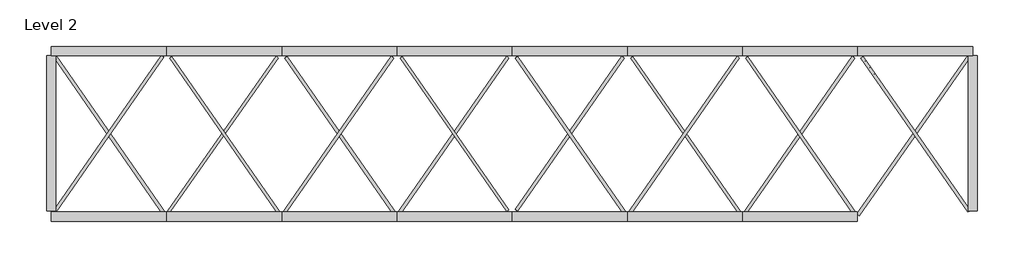
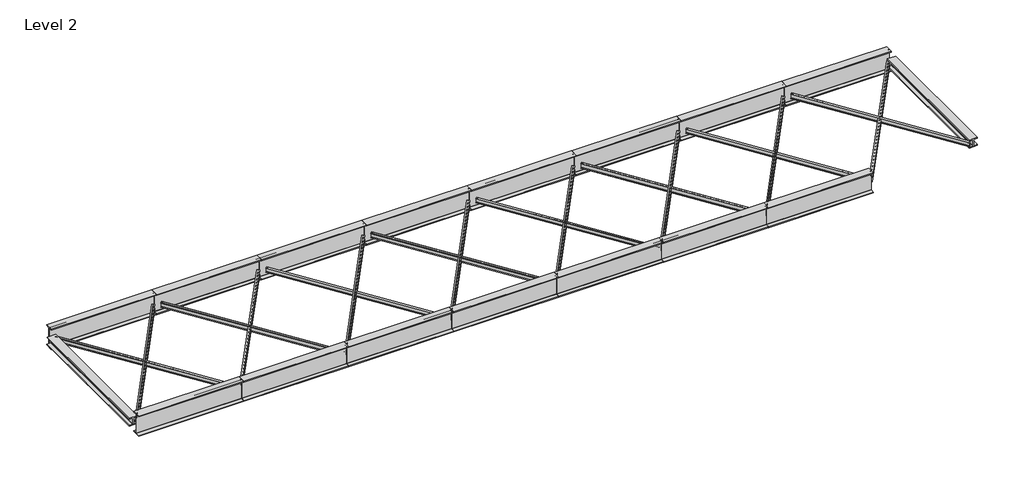
# One storey: 18 members, 15 beams.
"""IFC4 building model written with IfcOpenShell, lengths in millimetres."""

import ifcopenshell
import ifcopenshell.guid

model = None  # the IFC model being written
_history = None  # IfcOwnerHistory: only IFC2X3 demands one
_inside = {}  # id of a spatial element -> (the spatial element, [elements in it])
_under = {}  # id of a project, library or spatial element -> (it, [spatial elements below it])
_declared = {}  # id of a project -> (the project, [libraries it declares])
_typed = {}  # id of a type object -> (the type object, [elements of that type])
_made_of = {}  # id of a material, layer set ... -> (it, [elements and type objects made of it])


def new_model(schema):
    """Start an empty IFC model of exactly this schema.

    Asked for "IFC4X3", IfcOpenShell would pick the latest addendum, in which some entities
    have other attributes; the version numbers below select the first issue.
    IFC2X3 requires an IfcOwnerHistory on every rooted entity: one is made here for all.
    """
    global model, _history
    if schema == "IFC4X3":
        model = ifcopenshell.file(schema_version=(4, 3, 0, 0))
    else:
        model = ifcopenshell.file(schema=schema)
    _inside.clear()
    _under.clear()
    _declared.clear()
    _typed.clear()
    _made_of.clear()
    _history = None
    if model.schema == "IFC2X3":
        org = make("IfcOrganization", Name="unknown")
        user = make(
            "IfcPersonAndOrganization",
            ThePerson=make("IfcPerson", FamilyName="unknown"),
            TheOrganization=org,
        )
        app = make(
            "IfcApplication",
            ApplicationDeveloper=org,
            Version="unknown",
            ApplicationFullName="unknown",
            ApplicationIdentifier="unknown",
        )
        _history = make(
            "IfcOwnerHistory",
            OwningUser=user,
            OwningApplication=app,
            ChangeAction="ADDED",
            CreationDate=0,
        )
    return model


def make(cls, **values):
    """One entity of the class cls with the attributes given. An attribute that is None is left unset."""
    return model.create_entity(
        cls, **{name: value for name, value in values.items() if value is not None}
    )


def rooted(cls, **values):
    """An entity with a GlobalId (a new one), such as an element, a storey or a relation."""
    return make(cls, GlobalId=ifcopenshell.guid.new(), OwnerHistory=_history, **values)


def si_unit(unit_type, name, prefix=None):
    """IfcSIUnit, for example si_unit("LENGTHUNIT", "METRE", prefix="MILLI")."""
    return make("IfcSIUnit", UnitType=unit_type, Prefix=prefix, Name=name)


def assignment(units):
    """IfcUnitAssignment: the units of a project."""
    return None if units is None else make("IfcUnitAssignment", Units=units)


def point(xyz):
    """IfcCartesianPoint."""
    return None if xyz is None else make("IfcCartesianPoint", Coordinates=xyz)


def direction(xyz):
    """IfcDirection."""
    return None if xyz is None else make("IfcDirection", DirectionRatios=xyz)


def frame(location, z_axis=None, x_axis=None):
    """IfcAxis2Placement3D, a coordinate frame: its origin and axes. An axis left out is left unset."""
    return make(
        "IfcAxis2Placement3D",
        Location=point(location),
        Axis=direction(z_axis),
        RefDirection=direction(x_axis),
    )


def frame_2d(location, x_axis=None):
    """IfcAxis2Placement2D, a coordinate frame in the plane: its origin and x axis."""
    return make(
        "IfcAxis2Placement2D", Location=point(location), RefDirection=direction(x_axis)
    )


def origin():
    """The frame at (0, 0, 0) with its axes left unset."""
    return frame((0.0, 0.0, 0.0))


def place(relative_to, where):
    """IfcLocalPlacement: puts the frame where relative to a parent placement (None: the world)."""
    return make(
        "IfcLocalPlacement", PlacementRelTo=relative_to, RelativePlacement=where
    )


def context(
    kind, dimensions, precision=None, world=None, true_north=None, identifier=None
):
    """IfcGeometricRepresentationContext, for example the 3D "Model" context."""
    return make(
        "IfcGeometricRepresentationContext",
        ContextIdentifier=identifier,
        ContextType=kind,
        CoordinateSpaceDimension=dimensions,
        Precision=precision,
        WorldCoordinateSystem=world,
        TrueNorth=true_north,
    )


def project(units=None, contexts=None):
    """IfcProject with its units and contexts."""
    return rooted(
        "IfcProject",
        Name="project",
        RepresentationContexts=contexts,
        UnitsInContext=assignment(units),
    )


def spatial(cls, under=None, at=None, **own):
    """A site, building, storey or space (cls), placed at a placement, below another one or the project."""
    s = rooted(cls, ObjectPlacement=at, **own)
    if under is not None:
        _under.setdefault(under.id(), (under, []))[1].append(s)
    return s


def polyline(points):
    """IfcPolyline through the points."""
    return make("IfcPolyline", Points=[point(p) for p in points])


def circle_curve(where, radius):
    """IfcCircle in the frame where."""
    return make("IfcCircle", Position=where, Radius=radius)


def trimmed(basis, trim1, trim2, sense, master):
    """IfcTrimmedCurve: the piece of a basis curve between two trims."""
    return make(
        "IfcTrimmedCurve",
        BasisCurve=basis,
        Trim1=trim1,
        Trim2=trim2,
        SenseAgreement=sense,
        MasterRepresentation=master,
    )


def segment(curve, same_sense, transition):
    """IfcCompositeCurveSegment."""
    return make(
        "IfcCompositeCurveSegment",
        Transition=transition,
        SameSense=same_sense,
        ParentCurve=curve,
    )


def composite_curve(segments, self_intersect=None):
    """IfcCompositeCurve: segments joined end to end."""
    return make("IfcCompositeCurve", Segments=segments, SelfIntersect=self_intersect)


def outline(outer, holes=None, kind="AREA"):
    """IfcArbitraryClosedProfileDef: a profile drawn as a closed curve; with holes, ...WithVoids."""
    if holes is None:
        return make("IfcArbitraryClosedProfileDef", ProfileType=kind, OuterCurve=outer)
    return make(
        "IfcArbitraryProfileDefWithVoids",
        ProfileType=kind,
        OuterCurve=outer,
        InnerCurves=holes,
    )


def extrude(swept, where, along, depth):
    """IfcExtrudedAreaSolid: the profile swept, set in the frame where, extruded along a direction by depth."""
    return make(
        "IfcExtrudedAreaSolid",
        SweptArea=swept,
        Position=where,
        ExtrudedDirection=direction(along),
        Depth=depth,
    )


def shape(context_of_items, identifier, shape_type, items):
    """IfcShapeRepresentation: the items that make up one representation, for example the "Body"."""
    return make(
        "IfcShapeRepresentation",
        ContextOfItems=context_of_items,
        RepresentationIdentifier=identifier,
        RepresentationType=shape_type,
        Items=items,
    )


def source(mapping_origin, context_of_items, identifier, shape_type, items):
    """IfcRepresentationMap: a shape defined once, which mapped items show again and again."""
    return make(
        "IfcRepresentationMap",
        MappingOrigin=mapping_origin,
        MappedRepresentation=shape(context_of_items, identifier, shape_type, items),
    )


def transform(
    local_origin,
    x_axis=None,
    y_axis=None,
    z_axis=None,
    scale=None,
    scale2=None,
    scale3=None,
    uniform=True,
):
    """IfcCartesianTransformationOperator3D, or its non-uniform kind. x_axis, y_axis, z_axis: its Axis1, 2, 3."""
    if uniform:
        return make(
            "IfcCartesianTransformationOperator3D",
            Axis1=direction(x_axis),
            Axis2=direction(y_axis),
            LocalOrigin=point(local_origin),
            Scale=scale,
            Axis3=direction(z_axis),
        )
    return make(
        "IfcCartesianTransformationOperator3DnonUniform",
        Axis1=direction(x_axis),
        Axis2=direction(y_axis),
        LocalOrigin=point(local_origin),
        Scale=scale,
        Axis3=direction(z_axis),
        Scale2=scale2,
        Scale3=scale3,
    )


def mapped(mapping_source, mapping_target):
    """IfcMappedItem: shows the shape of a source again, moved by a transform."""
    return make(
        "IfcMappedItem", MappingSource=mapping_source, MappingTarget=mapping_target
    )


def made_of(thing, what):
    """Note that an element or type object is made of a material, layer set ...; save() writes the relation."""
    if what is not None:
        _made_of.setdefault(what.id(), (what, []))[1].append(thing)
    return thing


def element(
    cls,
    number,
    at=None,
    inside=None,
    cuts=None,
    type_object=None,
    material=None,
    context=None,
    identifier="Body",
    shape_type=None,
    held_by="IfcProductDefinitionShape",
    body=None,
    shapes=None,
    **own,
):
    """One element of the class cls, such as IfcWall. Its Tag is "e" and its number.

    at: its placement. inside: the storey or other place that contains it. cuts: it is an
    opening in that element (IfcRelVoidsElement). A single representation is given by context,
    identifier, shape_type and body (its items); several are given by shapes. held_by: the class
    of the entity that holds the representations. save() writes the other relations.
    """
    e = rooted(cls, Tag="e%d" % number, ObjectPlacement=at, **own)
    if body is not None:
        shapes = [shape(context, identifier, shape_type, body)]
    if shapes is not None:
        e.Representation = make(held_by, Representations=shapes)
    if inside is not None:
        _inside.setdefault(inside.id(), (inside, []))[1].append(e)
    if cuts is not None:
        rooted(
            "IfcRelVoidsElement", RelatingBuildingElement=cuts, RelatedOpeningElement=e
        )
    if type_object is not None:
        _typed.setdefault(type_object.id(), (type_object, []))[1].append(e)
    return made_of(e, material)


def aggregate(whole, parts):
    """IfcRelAggregates: a whole, such as a stair, and the parts it consists of."""
    return rooted("IfcRelAggregates", RelatingObject=whole, RelatedObjects=parts)


def save(model, path):
    """Write the relations noted so far, then the file.

    IfcRelAggregates (storeys below a building ...), IfcRelContainedInSpatialStructure (elements
    in a storey), IfcRelDefinesByType, IfcRelAssociatesMaterial and IfcRelDeclares: one each for
    every whole, place, type object, material and project.
    """
    for whole, parts in _under.values():
        aggregate(whole, parts)
    for where, things in _inside.values():
        rooted(
            "IfcRelContainedInSpatialStructure",
            RelatedElements=things,
            RelatingStructure=where,
        )
    for kind, things in _typed.values():
        rooted("IfcRelDefinesByType", RelatedObjects=things, RelatingType=kind)
    for what, things in _made_of.values():
        rooted("IfcRelAssociatesMaterial", RelatedObjects=things, RelatingMaterial=what)
    for by, libraries in _declared.values():
        rooted("IfcRelDeclares", RelatingContext=by, RelatedDefinitions=libraries)
    model.write(path)


def wwf_welded_wide_flange_wwf55x402_e03ff242(model_context):
    return source(origin(), model_context, "Body", "SweptSolid", [
        extrude(outline(polyline([(274.955, -649.986), (274.955, -700.024), (-274.955, -700.024), (-274.955, -649.986), (-19.05, -649.986), (-8.001, -638.937), (-8.001, 638.937), (-19.05, 649.986), (-274.955, 649.986), (-274.955, 700.024), (274.955, 700.024), (274.955, 649.986), (19.05, 649.986), (8.001, 638.937), (8.001, -638.937), (19.05, -649.986), (274.955, -649.986)])), frame((-3472.2183929, 0.0, 0.0), z_axis=(1.0, 0.0, 0.0), x_axis=(0.0, 1.0, 0.0)), (0.0, 0.0, 1.0), 6944.4367858),
    ])


def wwf_welded_wide_flange_wwf55x402_453157a7(model_context):
    return source(origin(), model_context, "Body", "SweptSolid", [
        extrude(outline(polyline([(274.955, -649.986), (274.955, -700.024), (-274.955, -700.024), (-274.955, -649.986), (-19.05, -649.986), (-8.001, -638.937), (-8.001, 638.937), (-19.05, 649.986), (-274.955, 649.986), (-274.955, 700.024), (274.955, 700.024), (274.955, 649.986), (19.05, 649.986), (8.001, 638.937), (8.001, -638.937), (19.05, -649.986), (274.955, -649.986)])), frame((-3472.218169, 0.0, 0.0), z_axis=(1.0, 0.0, 0.0), x_axis=(0.0, 1.0, 0.0)), (0.0, 0.0, 1.0), 6944.436338),
    ])


def wwf_welded_wide_flange_wwf55x402_a9ee8206(model_context):
    return source(origin(), model_context, "Body", "SweptSolid", [
        extrude(outline(polyline([(274.955, -649.986), (274.955, -700.024), (-274.955, -700.024), (-274.955, -649.986), (-19.05, -649.986), (-8.001, -638.937), (-8.001, 638.937), (-19.05, 649.986), (-274.955, 649.986), (-274.955, 700.024), (274.955, 700.024), (274.955, 649.986), (19.05, 649.986), (8.001, 638.937), (8.001, -638.937), (19.05, -649.986), (274.955, -649.986)])), frame((-3459.5263379, 0.0, 0.0), z_axis=(1.0, 0.0, 0.0), x_axis=(0.0, 1.0, 0.0)), (0.0, 0.0, 1.0), 6931.7526763),
    ])


def wwf_welded_wide_flange_wwf55x402_d8a73b6f(model_context):
    return source(origin(), model_context, "Body", "SweptSolid", [
        extrude(outline(polyline([(274.955, -649.986), (274.955, -700.024), (-274.955, -700.024), (-274.955, -649.986), (-19.05, -649.986), (-8.001, -638.937), (-8.001, 638.937), (-19.05, 649.986), (-274.955, 649.986), (-274.955, 700.024), (274.955, 700.024), (274.955, 649.986), (19.05, 649.986), (8.001, 638.937), (8.001, -638.937), (19.05, -649.986), (274.955, -649.986)])), frame((-3472.2200653, 0.0, 0.0), z_axis=(1.0, 0.0, 0.0), x_axis=(0.0, 1.0, 0.0)), (0.0, 0.0, 1.0), 6931.74013),
    ])


def wwf_welded_wide_flange_wwf55x402_ad15bced(model_context):
    return source(origin(), model_context, "Body", "SweptSolid", [
        extrude(outline(polyline([(274.955, -649.986), (274.955, -700.024), (-274.955, -700.024), (-274.955, -649.986), (-19.05, -649.986), (-8.001, -638.937), (-8.001, 638.937), (-19.05, 649.986), (-274.955, 649.986), (-274.955, 700.024), (274.955, 700.024), (274.955, 649.986), (19.05, 649.986), (8.001, 638.937), (8.001, -638.937), (19.05, -649.986), (274.955, -649.986)])), frame((-3459.52714, 0.0, 0.0), z_axis=(1.0, 0.0, 0.0), x_axis=(0.0, 1.0, 0.0)), (0.0, 0.0, 1.0), 6919.0542799),
    ])


def wwf_welded_wide_flange_wwf55x402_d46538ab(model_context):
    return source(origin(), model_context, "Body", "SweptSolid", [
        extrude(outline(polyline([(274.955, -649.986), (274.955, -700.024), (-274.955, -700.024), (-274.955, -649.986), (-19.05, -649.986), (-8.001, -638.937), (-8.001, 638.937), (-19.05, 649.986), (-274.955, 649.986), (-274.955, 700.024), (274.955, 700.024), (274.955, 649.986), (19.05, 649.986), (8.001, 638.937), (8.001, -638.937), (19.05, -649.986), (274.955, -649.986)])), frame((-3472.22503, 0.0, 0.0), z_axis=(1.0, 0.0, 0.0), x_axis=(0.0, 1.0, 0.0)), (0.0, 0.0, 1.0), 6931.7500593),
    ])


def wwf_welded_wide_flange_wwf55x402_6292d54f(model_context):
    return source(origin(), model_context, "Body", "SweptSolid", [
        extrude(outline(polyline([(274.955, -649.986), (274.955, -700.024), (-274.955, -700.024), (-274.955, -649.986), (-19.05, -649.986), (-8.001, -638.937), (-8.001, 638.937), (-19.05, 649.986), (-274.955, 649.986), (-274.955, 700.024), (274.955, 700.024), (274.955, 649.986), (19.05, 649.986), (8.001, 638.937), (8.001, -638.937), (19.05, -649.986), (274.955, -649.986)])), frame((-3472.2230903, 0.0, 0.0), z_axis=(1.0, 0.0, 0.0), x_axis=(0.0, 1.0, 0.0)), (0.0, 0.0, 1.0), 6931.7461799),
    ])


def wwf_welded_wide_flange_wwf55x402_e70519e9(model_context):
    return source(origin(), model_context, "Body", "SweptSolid", [
        extrude(outline(polyline([(274.955, -649.986), (274.955, -700.024), (-274.955, -700.024), (-274.955, -649.986), (-19.05, -649.986), (-8.001, -638.937), (-8.001, 638.937), (-19.05, 649.986), (-274.955, 649.986), (-274.955, 700.024), (274.955, 700.024), (274.955, 649.986), (19.05, 649.986), (8.001, 638.937), (8.001, -638.937), (19.05, -649.986), (274.955, -649.986)])), frame((-3459.5195507, 0.0, 0.0), z_axis=(1.0, 0.0, 0.0), x_axis=(0.0, 1.0, 0.0)), (0.0, 0.0, 1.0), 6931.739102),
    ])


def ub_universal_beams_ub305x165x40_783ac592(model_context):
    return source(origin(), model_context, "Body", "SweptSolid", [
        extrude(outline(composite_curve([segment(polyline([(82.5, -141.5), (82.5, -151.7), (-82.5, -151.7), (-82.5, -141.5), (-11.9, -141.5)]), True, "CONTINUOUS"), segment(trimmed(circle_curve(frame_2d((-11.9, -132.6)), 8.9), [point((-11.9, -141.5))], [point((-3.0, -132.6))], True, "CARTESIAN"), True, "CONTINUOUS"), segment(polyline([(-3.0, -132.6), (-3.0, 132.6)]), True, "CONTINUOUS"), segment(trimmed(circle_curve(frame_2d((-11.9, 132.6)), 8.9), [point((-3.0, 132.6))], [point((-11.9, 141.5))], True, "CARTESIAN"), True, "CONTINUOUS"), segment(polyline([(-11.9, 141.5), (-82.5, 141.5), (-82.5, 151.7), (82.5, 151.7), (82.5, 141.5), (11.9, 141.5)]), True, "CONTINUOUS"), segment(trimmed(circle_curve(frame_2d((11.9, 132.6)), 8.9), [point((11.9, 141.5))], [point((3.0, 132.6))], True, "CARTESIAN"), True, "CONTINUOUS"), segment(polyline([(3.0, 132.6), (3.0, -132.6)]), True, "CONTINUOUS"), segment(trimmed(circle_curve(frame_2d((11.9, -132.6)), 8.9), [point((3.0, -132.6))], [point((11.9, -141.5))], True, "CARTESIAN"), True, "CONTINUOUS"), segment(polyline([(11.9, -141.5), (82.5, -141.5)]), True, "CONTINUOUS")], self_intersect=False)), frame((-5697.7, 0.0, 0.0), z_axis=(1.0, 0.0, 0.0), x_axis=(0.0, 1.0, 0.0)), (0.0, 0.0, 1.0), 11670.0),
    ])


def ub_universal_beams_ub305x165x40_9e40c5b6(model_context):
    return source(origin(), model_context, "Body", "SweptSolid", [
        extrude(outline(composite_curve([segment(polyline([(82.5, -141.5), (82.5, -151.7), (-82.5, -151.7), (-82.5, -141.5), (-11.9, -141.5)]), True, "CONTINUOUS"), segment(trimmed(circle_curve(frame_2d((-11.9, -132.6)), 8.9), [point((-11.9, -141.5))], [point((-3.0, -132.6))], True, "CARTESIAN"), True, "CONTINUOUS"), segment(polyline([(-3.0, -132.6), (-3.0, 132.6)]), True, "CONTINUOUS"), segment(trimmed(circle_curve(frame_2d((-11.9, 132.6)), 8.9), [point((-3.0, 132.6))], [point((-11.9, 141.5))], True, "CARTESIAN"), True, "CONTINUOUS"), segment(polyline([(-11.9, 141.5), (-82.5, 141.5), (-82.5, 151.7), (82.5, 151.7), (82.5, 141.5), (11.9, 141.5)]), True, "CONTINUOUS"), segment(trimmed(circle_curve(frame_2d((11.9, 132.6)), 8.9), [point((11.9, 141.5))], [point((3.0, 132.6))], True, "CARTESIAN"), True, "CONTINUOUS"), segment(polyline([(3.0, 132.6), (3.0, -132.6)]), True, "CONTINUOUS"), segment(trimmed(circle_curve(frame_2d((11.9, -132.6)), 8.9), [point((3.0, -132.6))], [point((11.9, -141.5))], True, "CARTESIAN"), True, "CONTINUOUS"), segment(polyline([(11.9, -141.5), (82.5, -141.5)]), True, "CONTINUOUS")], self_intersect=False)), frame((-5682.6, 0.0, 0.0), z_axis=(1.0, 0.0, 0.0), x_axis=(0.0, 1.0, 0.0)), (0.0, 0.0, 1.0), 11365.2),
    ])


def ub_universal_beams_ub305x165x40_3335d084(model_context):
    return source(origin(), model_context, "Body", "SweptSolid", [
        extrude(outline(composite_curve([segment(polyline([(82.5, -141.5), (82.5, -151.7), (-82.5, -151.7), (-82.5, -141.5), (-11.9, -141.5)]), True, "CONTINUOUS"), segment(trimmed(circle_curve(frame_2d((-11.9, -132.6)), 8.9), [point((-11.9, -141.5))], [point((-3.0, -132.6))], True, "CARTESIAN"), True, "CONTINUOUS"), segment(polyline([(-3.0, -132.6), (-3.0, 132.6)]), True, "CONTINUOUS"), segment(trimmed(circle_curve(frame_2d((-11.9, 132.6)), 8.9), [point((-3.0, 132.6))], [point((-11.9, 141.5))], True, "CARTESIAN"), True, "CONTINUOUS"), segment(polyline([(-11.9, 141.5), (-82.5, 141.5), (-82.5, 151.7), (82.5, 151.7), (82.5, 141.5), (11.9, 141.5)]), True, "CONTINUOUS"), segment(trimmed(circle_curve(frame_2d((11.9, 132.6)), 8.9), [point((11.9, 141.5))], [point((3.0, 132.6))], True, "CARTESIAN"), True, "CONTINUOUS"), segment(polyline([(3.0, 132.6), (3.0, -132.6)]), True, "CONTINUOUS"), segment(trimmed(circle_curve(frame_2d((11.9, -132.6)), 8.9), [point((3.0, -132.6))], [point((11.9, -141.5))], True, "CARTESIAN"), True, "CONTINUOUS"), segment(polyline([(11.9, -141.5), (82.5, -141.5)]), True, "CONTINUOUS")], self_intersect=False)), frame((-5955.8, 0.0, 0.0), z_axis=(1.0, 0.0, 0.0), x_axis=(0.0, 1.0, 0.0)), (0.0, 0.0, 1.0), 11638.4),
    ])


def ub_universal_beams_ub305x165x40_035d116d(model_context):
    return source(origin(), model_context, "Body", "SweptSolid", [
        extrude(outline(composite_curve([segment(polyline([(82.5, -141.5), (82.5, -151.7), (-82.5, -151.7), (-82.5, -141.5), (-11.9, -141.5)]), True, "CONTINUOUS"), segment(trimmed(circle_curve(frame_2d((-11.9, -132.6)), 8.9), [point((-11.9, -141.5))], [point((-3.0, -132.6))], True, "CARTESIAN"), True, "CONTINUOUS"), segment(polyline([(-3.0, -132.6), (-3.0, 132.6)]), True, "CONTINUOUS"), segment(trimmed(circle_curve(frame_2d((-11.9, 132.6)), 8.9), [point((-3.0, 132.6))], [point((-11.9, 141.5))], True, "CARTESIAN"), True, "CONTINUOUS"), segment(polyline([(-11.9, 141.5), (-82.5, 141.5), (-82.5, 151.7), (82.5, 151.7), (82.5, 141.5), (11.9, 141.5)]), True, "CONTINUOUS"), segment(trimmed(circle_curve(frame_2d((11.9, 132.6)), 8.9), [point((11.9, 141.5))], [point((3.0, 132.6))], True, "CARTESIAN"), True, "CONTINUOUS"), segment(polyline([(3.0, 132.6), (3.0, -132.6)]), True, "CONTINUOUS"), segment(trimmed(circle_curve(frame_2d((11.9, -132.6)), 8.9), [point((3.0, -132.6))], [point((11.9, -141.5))], True, "CARTESIAN"), True, "CONTINUOUS"), segment(polyline([(11.9, -141.5), (82.5, -141.5)]), True, "CONTINUOUS")], self_intersect=False)), frame((-5621.65, 0.0, 0.0), z_axis=(1.0, 0.0, 0.0), x_axis=(0.0, 1.0, 0.0)), (0.0, 0.0, 1.0), 11577.5),
    ])


def ub_universal_beams_ub305x165x40_793367f0(model_context):
    return source(origin(), model_context, "Body", "SweptSolid", [
        extrude(outline(composite_curve([segment(polyline([(82.5, -141.5), (82.5, -151.7), (-82.5, -151.7), (-82.5, -141.5), (-11.9, -141.5)]), True, "CONTINUOUS"), segment(trimmed(circle_curve(frame_2d((-11.9, -132.6)), 8.9), [point((-11.9, -141.5))], [point((-3.0, -132.6))], True, "CARTESIAN"), True, "CONTINUOUS"), segment(polyline([(-3.0, -132.6), (-3.0, 132.6)]), True, "CONTINUOUS"), segment(trimmed(circle_curve(frame_2d((-11.9, 132.6)), 8.9), [point((-3.0, 132.6))], [point((-11.9, 141.5))], True, "CARTESIAN"), True, "CONTINUOUS"), segment(polyline([(-11.9, 141.5), (-82.5, 141.5), (-82.5, 151.7), (82.5, 151.7), (82.5, 141.5), (11.9, 141.5)]), True, "CONTINUOUS"), segment(trimmed(circle_curve(frame_2d((11.9, 132.6)), 8.9), [point((11.9, 141.5))], [point((3.0, 132.6))], True, "CARTESIAN"), True, "CONTINUOUS"), segment(polyline([(3.0, 132.6), (3.0, -132.6)]), True, "CONTINUOUS"), segment(trimmed(circle_curve(frame_2d((11.9, -132.6)), 8.9), [point((3.0, -132.6))], [point((11.9, -141.5))], True, "CARTESIAN"), True, "CONTINUOUS"), segment(polyline([(11.9, -141.5), (82.5, -141.5)]), True, "CONTINUOUS")], self_intersect=False)), frame((-5600.7, 0.0, 0.0), z_axis=(1.0, 0.0, 0.0), x_axis=(0.0, 1.0, 0.0)), (0.0, 0.0, 1.0), 11654.3),
    ])


def ub_universal_beams_ub305x165x40_c2663d37(model_context):
    return source(origin(), model_context, "Body", "SweptSolid", [
        extrude(outline(composite_curve([segment(polyline([(82.5, -141.5), (82.5, -151.7), (-82.5, -151.7), (-82.5, -141.5), (-11.9, -141.5)]), True, "CONTINUOUS"), segment(trimmed(circle_curve(frame_2d((-11.9, -132.6)), 8.9), [point((-11.9, -141.5))], [point((-3.0, -132.6))], True, "CARTESIAN"), True, "CONTINUOUS"), segment(polyline([(-3.0, -132.6), (-3.0, 132.6)]), True, "CONTINUOUS"), segment(trimmed(circle_curve(frame_2d((-11.9, 132.6)), 8.9), [point((-3.0, 132.6))], [point((-11.9, 141.5))], True, "CARTESIAN"), True, "CONTINUOUS"), segment(polyline([(-11.9, 141.5), (-82.5, 141.5), (-82.5, 151.7), (82.5, 151.7), (82.5, 141.5), (11.9, 141.5)]), True, "CONTINUOUS"), segment(trimmed(circle_curve(frame_2d((11.9, 132.6)), 8.9), [point((11.9, 141.5))], [point((3.0, 132.6))], True, "CARTESIAN"), True, "CONTINUOUS"), segment(polyline([(3.0, 132.6), (3.0, -132.6)]), True, "CONTINUOUS"), segment(trimmed(circle_curve(frame_2d((11.9, -132.6)), 8.9), [point((3.0, -132.6))], [point((11.9, -141.5))], True, "CARTESIAN"), True, "CONTINUOUS"), segment(polyline([(11.9, -141.5), (82.5, -141.5)]), True, "CONTINUOUS")], self_intersect=False)), frame((-5634.75, 0.0, 0.0), z_axis=(1.0, 0.0, 0.0), x_axis=(0.0, 1.0, 0.0)), (0.0, 0.0, 1.0), 11590.6),
    ])


def ub_universal_beams_ub305x165x40_eee0c611(model_context):
    return source(origin(), model_context, "Body", "SweptSolid", [
        extrude(outline(composite_curve([segment(polyline([(82.5, -141.5), (82.5, -151.7), (-82.5, -151.7), (-82.5, -141.5), (-11.9, -141.5)]), True, "CONTINUOUS"), segment(trimmed(circle_curve(frame_2d((-11.9, -132.6)), 8.9), [point((-11.9, -141.5))], [point((-3.0, -132.6))], True, "CARTESIAN"), True, "CONTINUOUS"), segment(polyline([(-3.0, -132.6), (-3.0, 132.6)]), True, "CONTINUOUS"), segment(trimmed(circle_curve(frame_2d((-11.9, 132.6)), 8.9), [point((-3.0, 132.6))], [point((-11.9, 141.5))], True, "CARTESIAN"), True, "CONTINUOUS"), segment(polyline([(-11.9, 141.5), (-82.5, 141.5), (-82.5, 151.7), (82.5, 151.7), (82.5, 141.5), (11.9, 141.5)]), True, "CONTINUOUS"), segment(trimmed(circle_curve(frame_2d((11.9, 132.6)), 8.9), [point((11.9, 141.5))], [point((3.0, 132.6))], True, "CARTESIAN"), True, "CONTINUOUS"), segment(polyline([(3.0, 132.6), (3.0, -132.6)]), True, "CONTINUOUS"), segment(trimmed(circle_curve(frame_2d((11.9, -132.6)), 8.9), [point((3.0, -132.6))], [point((11.9, -141.5))], True, "CARTESIAN"), True, "CONTINUOUS"), segment(polyline([(11.9, -141.5), (82.5, -141.5)]), True, "CONTINUOUS")], self_intersect=False)), frame((-5621.7, 0.0, 0.0), z_axis=(1.0, 0.0, 0.0), x_axis=(0.0, 1.0, 0.0)), (0.0, 0.0, 1.0), 11577.5),
    ])


def ub_universal_beams_ub305x165x40_8d2bc380(model_context):
    return source(origin(), model_context, "Body", "SweptSolid", [
        extrude(outline(composite_curve([segment(polyline([(82.5, -141.5), (82.5, -151.7), (-82.5, -151.7), (-82.5, -141.5), (-11.9, -141.5)]), True, "CONTINUOUS"), segment(trimmed(circle_curve(frame_2d((-11.9, -132.6)), 8.9), [point((-11.9, -141.5))], [point((-3.0, -132.6))], True, "CARTESIAN"), True, "CONTINUOUS"), segment(polyline([(-3.0, -132.6), (-3.0, 132.6)]), True, "CONTINUOUS"), segment(trimmed(circle_curve(frame_2d((-11.9, 132.6)), 8.9), [point((-3.0, 132.6))], [point((-11.9, 141.5))], True, "CARTESIAN"), True, "CONTINUOUS"), segment(polyline([(-11.9, 141.5), (-82.5, 141.5), (-82.5, 151.7), (82.5, 151.7), (82.5, 141.5), (11.9, 141.5)]), True, "CONTINUOUS"), segment(trimmed(circle_curve(frame_2d((11.9, 132.6)), 8.9), [point((11.9, 141.5))], [point((3.0, 132.6))], True, "CARTESIAN"), True, "CONTINUOUS"), segment(polyline([(3.0, 132.6), (3.0, -132.6)]), True, "CONTINUOUS"), segment(trimmed(circle_curve(frame_2d((11.9, -132.6)), 8.9), [point((3.0, -132.6))], [point((11.9, -141.5))], True, "CARTESIAN"), True, "CONTINUOUS"), segment(polyline([(11.9, -141.5), (82.5, -141.5)]), True, "CONTINUOUS")], self_intersect=False)), frame((-5621.7, 0.0, 0.0), z_axis=(1.0, 0.0, 0.0), x_axis=(0.0, 1.0, 0.0)), (0.0, 0.0, 1.0), 11256.5),
    ])


def ub_universal_beams_ub305x165x40_49d98a2e(model_context):
    return source(origin(), model_context, "Body", "SweptSolid", [
        extrude(outline(composite_curve([segment(polyline([(82.5, -141.5), (82.5, -151.7), (-82.5, -151.7), (-82.5, -141.5), (-11.9, -141.5)]), True, "CONTINUOUS"), segment(trimmed(circle_curve(frame_2d((-11.9, -132.6)), 8.9), [point((-11.9, -141.5))], [point((-3.0, -132.6))], True, "CARTESIAN"), True, "CONTINUOUS"), segment(polyline([(-3.0, -132.6), (-3.0, 132.6)]), True, "CONTINUOUS"), segment(trimmed(circle_curve(frame_2d((-11.9, 132.6)), 8.9), [point((-3.0, 132.6))], [point((-11.9, 141.5))], True, "CARTESIAN"), True, "CONTINUOUS"), segment(polyline([(-11.9, 141.5), (-82.5, 141.5), (-82.5, 151.7), (82.5, 151.7), (82.5, 141.5), (11.9, 141.5)]), True, "CONTINUOUS"), segment(trimmed(circle_curve(frame_2d((11.9, 132.6)), 8.9), [point((11.9, 141.5))], [point((3.0, 132.6))], True, "CARTESIAN"), True, "CONTINUOUS"), segment(polyline([(3.0, 132.6), (3.0, -132.6)]), True, "CONTINUOUS"), segment(trimmed(circle_curve(frame_2d((11.9, -132.6)), 8.9), [point((3.0, -132.6))], [point((11.9, -141.5))], True, "CARTESIAN"), True, "CONTINUOUS"), segment(polyline([(11.9, -141.5), (82.5, -141.5)]), True, "CONTINUOUS")], self_intersect=False)), frame((-5634.8, 0.0, 0.0), z_axis=(1.0, 0.0, 0.0), x_axis=(0.0, 1.0, 0.0)), (0.0, 0.0, 1.0), 11256.5),
    ])


def ub_universal_beams_ub305x165x40_967f8f3f(model_context):
    return source(origin(), model_context, "Body", "SweptSolid", [
        extrude(outline(composite_curve([segment(polyline([(82.5, -141.5), (82.5, -151.7), (-82.5, -151.7), (-82.5, -141.5), (-11.9, -141.5)]), True, "CONTINUOUS"), segment(trimmed(circle_curve(frame_2d((-11.9, -132.6)), 8.9), [point((-11.9, -141.5))], [point((-3.0, -132.6))], True, "CARTESIAN"), True, "CONTINUOUS"), segment(polyline([(-3.0, -132.6), (-3.0, 132.6)]), True, "CONTINUOUS"), segment(trimmed(circle_curve(frame_2d((-11.9, 132.6)), 8.9), [point((-3.0, 132.6))], [point((-11.9, 141.5))], True, "CARTESIAN"), True, "CONTINUOUS"), segment(polyline([(-11.9, 141.5), (-82.5, 141.5), (-82.5, 151.7), (82.5, 151.7), (82.5, 141.5), (11.9, 141.5)]), True, "CONTINUOUS"), segment(trimmed(circle_curve(frame_2d((11.9, 132.6)), 8.9), [point((11.9, 141.5))], [point((3.0, 132.6))], True, "CARTESIAN"), True, "CONTINUOUS"), segment(polyline([(3.0, 132.6), (3.0, -132.6)]), True, "CONTINUOUS"), segment(trimmed(circle_curve(frame_2d((11.9, -132.6)), 8.9), [point((3.0, -132.6))], [point((11.9, -141.5))], True, "CARTESIAN"), True, "CONTINUOUS"), segment(polyline([(11.9, -141.5), (82.5, -141.5)]), True, "CONTINUOUS")], self_intersect=False)), frame((-5621.7, 0.0, 0.0), z_axis=(1.0, 0.0, 0.0), x_axis=(0.0, 1.0, 0.0)), (0.0, 0.0, 1.0), 11304.3),
    ])


def ub_universal_beams_ub305x165x40_27ef7093(model_context):
    return source(origin(), model_context, "Body", "SweptSolid", [
        extrude(outline(composite_curve([segment(polyline([(82.5, -141.5), (82.5, -151.7), (-82.5, -151.7), (-82.5, -141.5), (-11.9, -141.5)]), True, "CONTINUOUS"), segment(trimmed(circle_curve(frame_2d((-11.9, -132.6)), 8.9), [point((-11.9, -141.5))], [point((-3.0, -132.6))], True, "CARTESIAN"), True, "CONTINUOUS"), segment(polyline([(-3.0, -132.6), (-3.0, 132.6)]), True, "CONTINUOUS"), segment(trimmed(circle_curve(frame_2d((-11.9, 132.6)), 8.9), [point((-3.0, 132.6))], [point((-11.9, 141.5))], True, "CARTESIAN"), True, "CONTINUOUS"), segment(polyline([(-11.9, 141.5), (-82.5, 141.5), (-82.5, 151.7), (82.5, 151.7), (82.5, 141.5), (11.9, 141.5)]), True, "CONTINUOUS"), segment(trimmed(circle_curve(frame_2d((11.9, 132.6)), 8.9), [point((11.9, 141.5))], [point((3.0, 132.6))], True, "CARTESIAN"), True, "CONTINUOUS"), segment(polyline([(3.0, 132.6), (3.0, -132.6)]), True, "CONTINUOUS"), segment(trimmed(circle_curve(frame_2d((11.9, -132.6)), 8.9), [point((3.0, -132.6))], [point((11.9, -141.5))], True, "CARTESIAN"), True, "CONTINUOUS"), segment(polyline([(11.9, -141.5), (82.5, -141.5)]), True, "CONTINUOUS")], self_intersect=False)), frame((-5606.85, 0.0, 0.0), z_axis=(1.0, 0.0, 0.0), x_axis=(0.0, 1.0, 0.0)), (0.0, 0.0, 1.0), 11546.3),
    ])


def wwf_welded_wide_flange_wwf22x484_0dac382b(model_context):
    return source(origin(), model_context, "Body", "SweptSolid", [
        extrude(outline(polyline([(274.955, -214.9602), (274.955, -274.955), (-274.955, -274.955), (-274.955, -214.9602), (-47.625, -214.9602), (-29.9974, -197.3326), (-29.9974, 197.3326), (-47.625, 214.9602), (-274.955, 214.9602), (-274.955, 274.955), (274.955, 274.955), (274.955, 214.9602), (47.625, 214.9602), (29.9974, 197.3326), (29.9974, -197.3326), (47.625, -214.9602), (274.955, -214.9602)])), frame((-4712.345, 0.0, 0.0), z_axis=(1.0, 0.0, 0.0), x_axis=(0.0, 1.0, 0.0)), (0.0, 0.0, 1.0), 9374.652),
    ])


model = new_model("IFC4")

# Units and contexts
model_context = context("Model", 3, world=origin())
ifc_project = project(units=[si_unit("LENGTHUNIT", "METRE", prefix="MILLI")], contexts=[model_context])

# Site, building, storey
site = spatial("IfcSite", under=ifc_project)
building = spatial("IfcBuilding", under=site)
storey = spatial("IfcBuildingStorey", under=building, Name="Level 2", Elevation=9000.0)

# Beams
placement = place(None, origin())
wwf_welded_wide_flange_wwf55x402_shape = wwf_welded_wide_flange_wwf55x402_e03ff242(model_context)
element("IfcBeam", 1, ObjectType="WWF-Welded Wide Flange : WWF55x402", at=placement, inside=storey, context=model_context, shape_type="MappedRepresentation", body=[
    mapped(wwf_welded_wide_flange_wwf55x402_shape, transform((71453.5176866, -42624.2714806, 9000.0), x_axis=(-1.0, 0.0, 0.0), y_axis=(0.0, -1.0, 0.0), z_axis=(0.0, 0.0, 1.0))),
])
wwf_welded_wide_flange_wwf55x402_2_shape = wwf_welded_wide_flange_wwf55x402_453157a7(model_context)
element("IfcBeam", 2, ObjectType="WWF-Welded Wide Flange : WWF55x402", at=placement, inside=storey, context=model_context, shape_type="MappedRepresentation", body=[
    mapped(wwf_welded_wide_flange_wwf55x402_2_shape, transform((22842.398693, -52624.2714806, 9000.0), x_axis=(-1.0, 0.0, 0.0), y_axis=(0.0, -1.0, 0.0), z_axis=(0.0, 0.0, 1.0))),
])
element("IfcBeam", 3, ObjectType="WWF-Welded Wide Flange : WWF55x402", at=placement, inside=storey, context=model_context, shape_type="MappedRepresentation", body=[
    mapped(wwf_welded_wide_flange_wwf55x402_2_shape, transform((22842.398693, -42624.2714806, 9000.0), x_axis=(-1.0, 0.0, 0.0), y_axis=(0.0, -1.0, 0.0), z_axis=(0.0, 0.0, 1.0))),
])
wwf_welded_wide_flange_wwf55x402_3_shape = wwf_welded_wide_flange_wwf55x402_a9ee8206(model_context)
element("IfcBeam", 4, ObjectType="WWF-Welded Wide Flange : WWF55x402", at=placement, inside=storey, context=model_context, shape_type="MappedRepresentation", body=[
    mapped(wwf_welded_wide_flange_wwf55x402_3_shape, transform((57564.6338526, -52624.2714806, 9000.0), x_axis=(-1.0, 0.0, 0.0), y_axis=(0.0, -1.0, 0.0), z_axis=(0.0, 0.0, 1.0))),
])
element("IfcBeam", 5, ObjectType="WWF-Welded Wide Flange : WWF55x402", at=placement, inside=storey, context=model_context, shape_type="MappedRepresentation", body=[
    mapped(wwf_welded_wide_flange_wwf55x402_3_shape, transform((57564.6338526, -42624.2714806, 9000.0), x_axis=(-1.0, 0.0, 0.0), y_axis=(0.0, -1.0, 0.0), z_axis=(0.0, 0.0, 1.0))),
])
wwf_welded_wide_flange_wwf55x402_4_shape = wwf_welded_wide_flange_wwf55x402_d8a73b6f(model_context)
element("IfcBeam", 6, ObjectType="WWF-Welded Wide Flange : WWF55x402", at=placement, inside=storey, context=model_context, shape_type="MappedRepresentation", body=[
    mapped(wwf_welded_wide_flange_wwf55x402_4_shape, transform((29786.8369272, -52624.2714806, 9000.0), x_axis=(-1.0, 0.0, 0.0), y_axis=(0.0, -1.0, 0.0), z_axis=(0.0, 0.0, 1.0))),
])
element("IfcBeam", 7, ObjectType="WWF-Welded Wide Flange : WWF55x402", at=placement, inside=storey, context=model_context, shape_type="MappedRepresentation", body=[
    mapped(wwf_welded_wide_flange_wwf55x402_4_shape, transform((29786.8369272, -42624.2714806, 9000.0), x_axis=(-1.0, 0.0, 0.0), y_axis=(0.0, -1.0, 0.0), z_axis=(0.0, 0.0, 1.0))),
])
wwf_welded_wide_flange_wwf55x402_5_shape = wwf_welded_wide_flange_wwf55x402_ad15bced(model_context)
element("IfcBeam", 8, ObjectType="WWF-Welded Wide Flange : WWF55x402", at=placement, inside=storey, context=model_context, shape_type="MappedRepresentation", body=[
    mapped(wwf_welded_wide_flange_wwf55x402_5_shape, transform((50620.1803736, -52624.2714806, 9000.0), x_axis=(-1.0, 0.0, 0.0), y_axis=(0.0, -1.0, 0.0), z_axis=(0.0, 0.0, 1.0))),
])
element("IfcBeam", 9, ObjectType="WWF-Welded Wide Flange : WWF55x402", at=placement, inside=storey, context=model_context, shape_type="MappedRepresentation", body=[
    mapped(wwf_welded_wide_flange_wwf55x402_5_shape, transform((50620.1803736, -42624.2714806, 9000.0), x_axis=(-1.0, 0.0, 0.0), y_axis=(0.0, -1.0, 0.0), z_axis=(0.0, 0.0, 1.0))),
])
wwf_welded_wide_flange_wwf55x402_6_shape = wwf_welded_wide_flange_wwf55x402_d46538ab(model_context)
element("IfcBeam", 10, ObjectType="WWF-Welded Wide Flange : WWF55x402", at=placement, inside=storey, context=model_context, shape_type="MappedRepresentation", body=[
    mapped(wwf_welded_wide_flange_wwf55x402_6_shape, transform((43675.728203, -52624.2714806, 9000.0), x_axis=(-1.0, 0.0, 0.0), y_axis=(0.0, -1.0, 0.0), z_axis=(0.0, 0.0, 1.0))),
])
element("IfcBeam", 11, ObjectType="WWF-Welded Wide Flange : WWF55x402", at=placement, inside=storey, context=model_context, shape_type="MappedRepresentation", body=[
    mapped(wwf_welded_wide_flange_wwf55x402_6_shape, transform((43675.728203, -42624.2714806, 9000.0), x_axis=(-1.0, 0.0, 0.0), y_axis=(0.0, -1.0, 0.0), z_axis=(0.0, 0.0, 1.0))),
])
wwf_welded_wide_flange_wwf55x402_7_shape = wwf_welded_wide_flange_wwf55x402_6292d54f(model_context)
element("IfcBeam", 12, ObjectType="WWF-Welded Wide Flange : WWF55x402", at=placement, inside=storey, context=model_context, shape_type="MappedRepresentation", body=[
    mapped(wwf_welded_wide_flange_wwf55x402_7_shape, transform((36731.2800828, -52624.2714806, 9000.0), x_axis=(-1.0, 0.0, 0.0), y_axis=(0.0, -1.0, 0.0), z_axis=(0.0, 0.0, 1.0))),
])
element("IfcBeam", 13, ObjectType="WWF-Welded Wide Flange : WWF55x402", at=placement, inside=storey, context=model_context, shape_type="MappedRepresentation", body=[
    mapped(wwf_welded_wide_flange_wwf55x402_7_shape, transform((36731.2800828, -42624.2714806, 9000.0), x_axis=(-1.0, 0.0, 0.0), y_axis=(0.0, -1.0, 0.0), z_axis=(0.0, 0.0, 1.0))),
])
wwf_welded_wide_flange_wwf55x402_8_shape = wwf_welded_wide_flange_wwf55x402_e70519e9(model_context)
element("IfcBeam", 14, ObjectType="WWF-Welded Wide Flange : WWF55x402", at=placement, inside=storey, context=model_context, shape_type="MappedRepresentation", body=[
    mapped(wwf_welded_wide_flange_wwf55x402_8_shape, transform((64509.0797424, -52624.2714806, 9000.0), x_axis=(-1.0, 0.0, 0.0), y_axis=(0.0, -1.0, 0.0), z_axis=(0.0, 0.0, 1.0))),
])
element("IfcBeam", 15, ObjectType="WWF-Welded Wide Flange : WWF55x402", at=placement, inside=storey, context=model_context, shape_type="MappedRepresentation", body=[
    mapped(wwf_welded_wide_flange_wwf55x402_8_shape, transform((64509.0797424, -42624.2714806, 9000.0), x_axis=(-1.0, 0.0, 0.0), y_axis=(0.0, -1.0, 0.0), z_axis=(0.0, 0.0, 1.0))),
])

# Members
ub_universal_beams_ub305x165x40_shape = ub_universal_beams_ub305x165x40_783ac592(model_context)
element("IfcMember", 16, ObjectType="UB-Universal Beams : UB305x165x40", at=placement, inside=storey, context=model_context, shape_type="MappedRepresentation", body=[
    mapped(ub_universal_beams_ub305x165x40_shape, transform((71424.6706107, -47624.2714806, 9000.0), x_axis=(-0.5735764363510522, -0.8191520442889876, 0.0), y_axis=(0.8191520442889875, -0.5735764363510523, 0.0), z_axis=(0.0, 0.0, 1.0))),
])
ub_universal_beams_ub305x165x40_2_shape = ub_universal_beams_ub305x165x40_9e40c5b6(model_context)
element("IfcMember", 17, ObjectType="UB-Universal Beams : UB305x165x40", at=placement, inside=storey, context=model_context, shape_type="MappedRepresentation", body=[
    mapped(ub_universal_beams_ub305x165x40_2_shape, transform((22842.398693, -47624.2714806, 9000.0), x_axis=(0.5703933466604793, 0.8213716759698123, 0.0), y_axis=(-0.8213716759698123, 0.5703933466604793, 0.0), z_axis=(0.0, 0.0, 1.0))),
])
ub_universal_beams_ub305x165x40_3_shape = ub_universal_beams_ub305x165x40_3335d084(model_context)
element("IfcMember", 18, ObjectType="UB-Universal Beams : UB305x165x40", at=placement, inside=storey, context=model_context, shape_type="MappedRepresentation", body=[
    mapped(ub_universal_beams_ub305x165x40_3_shape, transform((22842.4178101, -47624.2714806, 9000.0), x_axis=(-0.5703954653672857, 0.8213702046510074, 0.0), y_axis=(-0.8213702046510072, -0.5703954653672858, 0.0), z_axis=(0.0, 0.0, 1.0))),
])
ub_universal_beams_ub305x165x40_4_shape = ub_universal_beams_ub305x165x40_035d116d(model_context)
element("IfcMember", 19, ObjectType="UB-Universal Beams : UB305x165x40", at=placement, inside=storey, context=model_context, shape_type="MappedRepresentation", body=[
    mapped(ub_universal_beams_ub305x165x40_4_shape, transform((29786.8612114, -47624.2714806, 8999.999302), x_axis=(0.5703973036870466, -0.8213689280381467, 1.1466695138396799e-07), y_axis=(0.8213689280381519, 0.5703973036870505, 0.0), z_axis=(-6.540571843238511e-08, 9.418387195288184e-08, 0.9999999999999936))),
])
ub_universal_beams_ub305x165x40_5_shape = ub_universal_beams_ub305x165x40_793367f0(model_context)
element("IfcMember", 20, ObjectType="UB-Universal Beams : UB305x165x40", at=placement, inside=storey, context=model_context, shape_type="MappedRepresentation", body=[
    mapped(ub_universal_beams_ub305x165x40_5_shape, transform((29786.8650157, -47583.115453, 8999.995382), x_axis=(-0.5735751095585876, -0.8191529733171163, 7.628491374143794e-07), y_axis=(0.8191529733173546, -0.5735751095587545, 0.0), z_axis=(4.37551279024362e-07, 6.24890138086694e-07, 0.9999999999997089))),
])
ub_universal_beams_ub305x165x40_6_shape = ub_universal_beams_ub305x165x40_c2663d37(model_context)
element("IfcMember", 21, ObjectType="UB-Universal Beams : UB305x165x40", at=placement, inside=storey, context=model_context, shape_type="MappedRepresentation", body=[
    mapped(ub_universal_beams_ub305x165x40_6_shape, transform((36731.3068713, -47624.2714806, 8999.9961517), x_axis=(-0.5703944499975186, -0.8213709097670969, 6.321820471067611e-07), y_axis=(0.8213709097672608, -0.5703944499976331, 0.0), z_axis=(3.605931325168864e-07, 5.192559421573857e-07, 0.9999999999998002))),
])
ub_universal_beams_ub305x165x40_7_shape = ub_universal_beams_ub305x165x40_eee0c611(model_context)
element("IfcMember", 22, ObjectType="UB-Universal Beams : UB305x165x40", at=placement, inside=storey, context=model_context, shape_type="MappedRepresentation", body=[
    mapped(ub_universal_beams_ub305x165x40_7_shape, transform((36731.3048763, -47624.2714806, 8999.995382), x_axis=(0.5703968820733968, -0.8213692208260376, 7.586168963547257e-07), y_axis=(0.8213692208262741, 0.5703968820735607, 0.0), z_axis=(-4.3271271091001233e-07, 6.231045700777557e-07, 0.9999999999997122))),
])
ub_universal_beams_ub305x165x40_8_shape = ub_universal_beams_ub305x165x40_8d2bc380(model_context)
element("IfcMember", 23, ObjectType="UB-Universal Beams : UB305x165x40", at=placement, inside=storey, context=model_context, shape_type="MappedRepresentation", body=[
    mapped(ub_universal_beams_ub305x165x40_8_shape, transform((43675.7362719, -47624.2714806, 8999.9995014), x_axis=(0.5703957881769911, -0.8213699804777033, 8.190506997962623e-08), y_axis=(0.8213699804777062, 0.5703957881769927, 0.0), z_axis=(-4.671830548767448e-08, 6.727436674341721e-08, 0.9999999999999969))),
])
element("IfcMember", 24, ObjectType="UB-Universal Beams : UB305x165x40", at=placement, inside=storey, context=model_context, shape_type="MappedRepresentation", body=[
    mapped(ub_universal_beams_ub305x165x40_6_shape, transform((43675.7475391, -47624.2714806, 9000.0), x_axis=(-0.5703945394597881, -0.8213708476409765, 0.0), y_axis=(0.8213708476409766, -0.5703945394597879, 0.0), z_axis=(0.0, 0.0, 1.0))),
])
element("IfcMember", 25, ObjectType="UB-Universal Beams : UB305x165x40", at=placement, inside=storey, context=model_context, shape_type="MappedRepresentation", body=[
    mapped(ub_universal_beams_ub305x165x40_4_shape, transform((50620.1873997, -47624.2714806, 9000.0), x_axis=(0.5703965715147088, -0.8213694364926576, 0.0), y_axis=(0.8213694364926575, 0.570396571514709, 0.0), z_axis=(0.0, 0.0, 1.0000000000000002))),
])
ub_universal_beams_ub305x165x40_9_shape = ub_universal_beams_ub305x165x40_49d98a2e(model_context)
element("IfcMember", 26, ObjectType="UB-Universal Beams : UB305x165x40", at=placement, inside=storey, context=model_context, shape_type="MappedRepresentation", body=[
    mapped(ub_universal_beams_ub305x165x40_9_shape, transform((50620.1814148, -47624.2714806, 8999.997691), x_axis=(-0.5703959082222089, -0.8213698971128768, 3.7930875999755814e-07), y_axis=(0.8213698971129362, -0.5703959082222493, 0.0), z_axis=(2.1635616611450859e-07, 3.1155279616000287e-07, 0.9999999999999282))),
])
ub_universal_beams_ub305x165x40_10_shape = ub_universal_beams_ub305x165x40_967f8f3f(model_context)
element("IfcMember", 27, ObjectType="UB-Universal Beams : UB305x165x40", at=placement, inside=storey, context=model_context, shape_type="MappedRepresentation", body=[
    mapped(ub_universal_beams_ub305x165x40_10_shape, transform((71453.5002654, -47624.2714806, 8999.9992303), x_axis=(0.5703942373162557, -0.8213710574620894, 1.2643643091133146e-07), y_axis=(0.8213710574620959, 0.5703942373162602, 0.0), z_axis=(-7.211861011961083e-08, 1.0385122597259727e-07, 0.999999999999992))),
])
ub_universal_beams_ub305x165x40_11_shape = ub_universal_beams_ub305x165x40_27ef7093(model_context)
element("IfcMember", 28, ObjectType="UB-Universal Beams : UB305x165x40", at=placement, inside=storey, context=model_context, shape_type="MappedRepresentation", body=[
    mapped(ub_universal_beams_ub305x165x40_11_shape, transform((64480.240649, -47624.2714806, 8999.9984607), x_axis=(0.5671876966090929, -0.8235885603960315, 2.5355555900284363e-07), y_axis=(0.823588560396058, 0.5671876966091108, 0.0), z_axis=(-1.4381359201027125e-07, 2.0882545882709746e-07, 0.999999999999968))),
])
element("IfcMember", 29, ObjectType="UB-Universal Beams : UB305x165x40", at=placement, inside=storey, context=model_context, shape_type="MappedRepresentation", body=[
    mapped(ub_universal_beams_ub305x165x40_6_shape, transform((64509.0742936, -47624.2714806, 8999.9992303), x_axis=(-0.570395334390623, -0.8213702956069167, 1.2643631363638412e-07), y_axis=(0.8213702956069233, -0.5703953343906271, 0.0), z_axis=(7.211868485479029e-08, 1.0385103129374081e-07, 0.999999999999992))),
])
element("IfcMember", 30, ObjectType="UB-Universal Beams : UB305x165x40", at=placement, inside=storey, context=model_context, shape_type="MappedRepresentation", body=[
    mapped(ub_universal_beams_ub305x165x40_6_shape, transform((57564.6319211, -47624.2714806, 8999.9998006), x_axis=(-0.5703950560018562, -0.8213704889321494, 3.276204807692467e-08), y_axis=(0.8213704889321498, -0.5703950560018567, 0.0), z_axis=(1.868731170662005e-08, 2.6909778434137055e-08, 0.9999999999999994))),
])
element("IfcMember", 31, ObjectType="UB-Universal Beams : UB305x165x40", at=placement, inside=storey, context=model_context, shape_type="MappedRepresentation", body=[
    mapped(ub_universal_beams_ub305x165x40_7_shape, transform((57564.6304431, -47624.2714806, 8999.997691), x_axis=(0.570396218781573, -0.8213696814465092, 3.7930866040278744e-07), y_axis=(0.8213696814465682, 0.5703962187816142, 0.0), z_axis=(-2.1635622418582365e-07, 3.1155263457818933e-07, 0.9999999999999281))),
])
wwf_welded_wide_flange_wwf22x484_shape = wwf_welded_wide_flange_wwf22x484_0dac382b(model_context)
element("IfcMember", 32, ObjectType="WWF-Welded Wide Flange : WWF22x484", at=placement, inside=storey, context=model_context, shape_type="MappedRepresentation", body=[
    mapped(wwf_welded_wide_flange_wwf22x484_shape, transform((74925.7360795, -47624.2714806, 9000.0), x_axis=(0.0, -1.0, 0.0), y_axis=(1.0, 0.0, 0.0), z_axis=(0.0, 0.0, 1.0))),
])
element("IfcMember", 33, ObjectType="WWF-Welded Wide Flange : WWF22x484", at=placement, inside=storey, context=model_context, shape_type="MappedRepresentation", body=[
    mapped(wwf_welded_wide_flange_wwf22x484_shape, transform((19370.180524, -47624.2714806, 9000.0), x_axis=(0.0, -1.0, 0.0), y_axis=(1.0, 0.0, 0.0), z_axis=(0.0, 0.0, 1.0))),
])

save(model, "model.ifc")

# Revit data of these elements
# Project information
#   Project Issue Date = "Issue Date"
#   Project Status = "Project Status"
#   Client Name = "Owner"
#   Project Address = "Enter address here"
#   Project Name = "Project Name"
#   Project Number = "Project Number"
# Grids (mm)
#   "4": line (78397.958, -34695.242) -> (78397.958, -52624.271)
#   "12": line (71453.514, -34695.242) -> (71453.514, -52624.271)
#   "13": line (64509.069, -34695.242) -> (64509.069, -52624.271)
#   "14": line (50620.181, -34695.242) -> (50620.181, -52624.271)
#   "15": line (43675.736, -34695.242) -> (43675.736, -52624.271)
#   "16": line (36731.292, -34695.242) -> (36731.292, -52624.271)
#   "17": line (29786.847, -34695.242) -> (29786.847, -52624.271)
#   "18": line (15897.958, -34695.242) -> (15897.958, -52624.271)
#   "19": line (57564.625, -34695.242) -> (57564.625, -52624.271)
#   "20": line (22842.403, -34695.242) -> (22842.403, -52624.271)
# Type "WWF-Welded Wide Flange : WWF55x402"
#   Assembly Code = "B10"
#   Nominal d = "12"
#   W = 402
#   Length [instance default] = 1524 mm
#   bf = 549.91 mm
#   d = 1400.048 mm
#   k = 19.05 mm
#   tf = 50.038 mm
#   tw = 16.002 mm
#   A = 0.0761289 m²
#   Structural Material [instance default] = Steel ASTM A572
# Type "UB-Universal Beams : UB305x165x40"
#   Section Name Key = "UB305X165X40"
#   Width = 16.5 cm
#   Web Thickness = 0.6 cm
#   Web Fillet = 0.89 cm
#   Warping Constant = 164000.0 cm⁶
#   Torsional Moment of Inertia = 14.70 cm⁴
#   Section Area = 51.3 cm²
#   Plastic Modulus weak axis = 142.0 cm³
#   Plastic Modulus strong axis = 623.0 cm³
#   Nominal Weight = 40.2999 kgf/m
#   Moment of Inertia weak axis = 764.00 cm⁴
#   Moment of Inertia strong axis = 8503.00 cm⁴
#   Height = 30.34 cm
#   Flange Thickness = 1.02 cm
#   Elastic Modulus weak axis = 92.6 cm³
#   Elastic Modulus strong axis = 560.0 cm³
#   Centroid Vertical = 15.17 cm
#   Centroid Horizontal = 8.25 cm
#   Bolt Spacing = 9.0 cm
#   Length [instance default] = 1500 mm
#   Structural Material [instance default] = Metal - Steel 43-275
#   Type Comments = ""
#   Assembly Code = ""
# Type "WWF-Welded Wide Flange : WWF22x484"
#   Assembly Code = "B10"
#   Nominal d = "12"
#   W = 484
#   Length [instance default] = 1524 mm
#   bf = 549.91 mm
#   d = 549.91 mm
#   k = 47.625 mm
#   tf = 59.995 mm
#   tw = 59.995 mm
#   A = 0.0922579 m²
#   Structural Material [instance default] = Steel ASTM A572
# Elements 1, 2, 3, 4, 5, 6, 7, 8, 9, 10, 11, 12, 13, 14, 15 (IfcBeam, "WWF-Welded Wide Flange : WWF55x402")
#   Structural Material = Metal - Steel 43-275
#   Phase Created = New Construction
#   Materials on its faces: "Metal - Steel 43-275"
# Elements 16, 17, 18, 19, 20, 21, 22, 23, 24, 25, 26, 27, 28, 29, 30, 31 (IfcMember, "UB-Universal Beams : UB305x165x40")
#   Structural Material = Metal - Steel 43-275
#   Phase Created = New Construction
#   Materials on its faces: "Metal - Steel 43-275"
# Elements 32, 33 (IfcMember, "WWF-Welded Wide Flange : WWF22x484")
#   Structural Material = Steel ASTM A572
#   Phase Created = New Construction
#   Materials on its faces: "Steel ASTM A572"
# Materials
#   "Steel ASTM A572": class "Metal", colour RGB 247 247 247, transparency 0, Description = "Structural steel, high strength low alloy, ASTM - A572 - 50", Cost = 0
#   "Metal - Steel 43-275": class "Metal", colour RGB 247 247 247, transparency 0, Cost = 0
